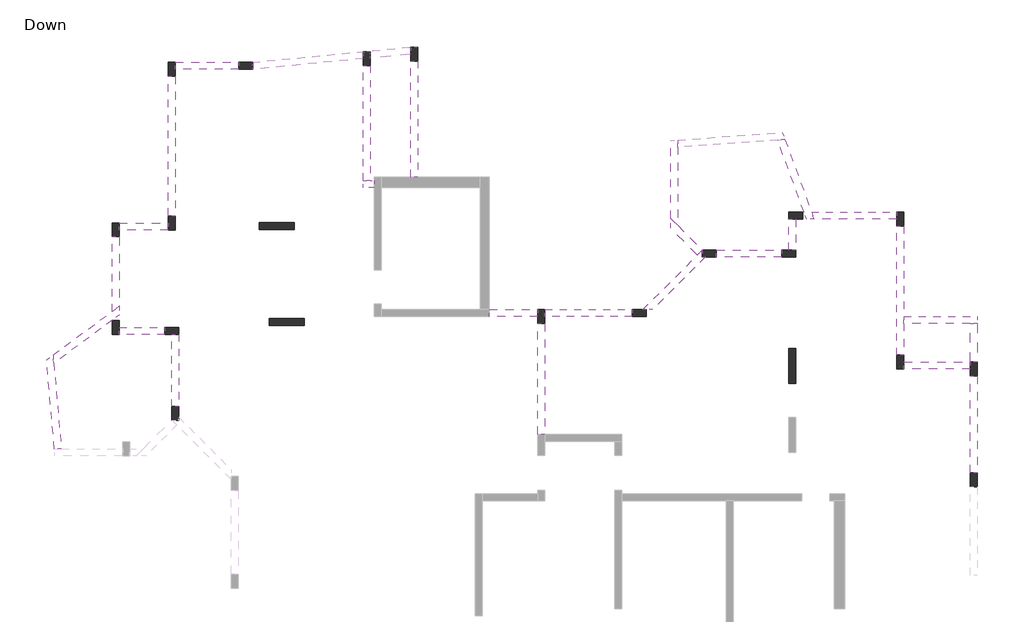
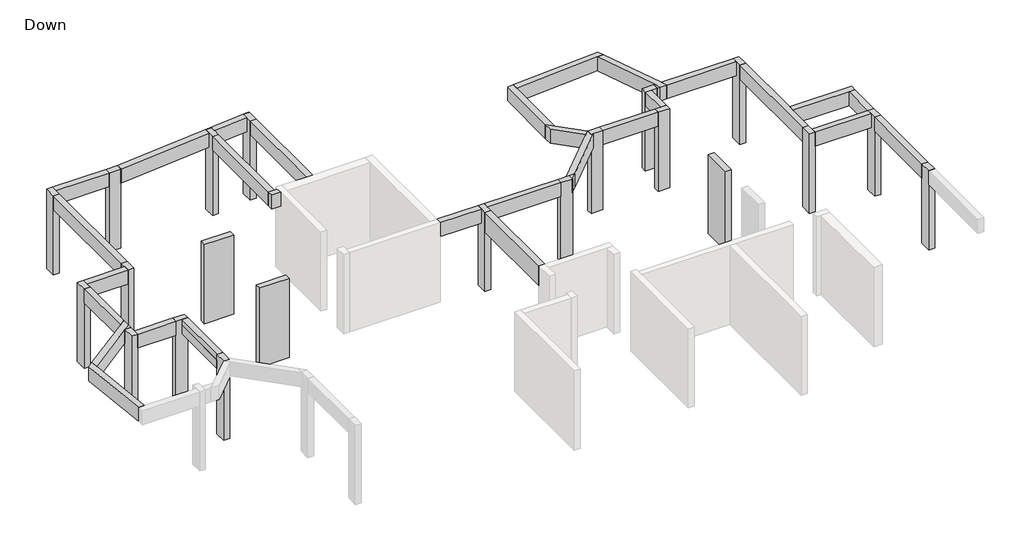
# One storey, part 3 of 3: 28 beams, 21 columns.
# Revit data of these elements (continued)
# Element 43 (IfcColumn, "Concrete Rectengular Column : 20/40") (continued)
#   Materials on its faces: "Concrete"
# Element 44 (IfcColumn, "Concrete Rectengular Column : 20/40")
#   Comments = ""
#   Mark = "C42"
#   SOFiSTiK_AMG_Comments = ""
#   SOFiSTiK_AMG_Scheduled = yes
#   SOFiSTiK_AMG_Adjusted = yes
#   Structural Material = Concrete
#   Phase Created = New Construction
#   Materials on its faces: "Concrete"
# Element 45 (IfcColumn, "Concrete Rectengular Column : 20/40")
#   Comments = ""
#   Mark = "C43"
#   SOFiSTiK_AMG_Comments = ""
#   SOFiSTiK_AMG_Scheduled = yes
#   SOFiSTiK_AMG_Adjusted = yes
#   Structural Material = Concrete
#   Phase Created = New Construction
#   Materials on its faces: "Concrete"
# Element 46 (IfcColumn, "Concrete Rectengular Column : 20/40")
#   Comments = ""
#   Mark = "C44"
#   SOFiSTiK_AMG_Comments = ""
#   SOFiSTiK_AMG_Scheduled = yes
#   SOFiSTiK_AMG_Adjusted = yes
#   Structural Material = Concrete
#   Phase Created = New Construction
#   Materials on its faces: "Concrete"
# Element 47 (IfcColumn, "Concrete Rectengular Column : 20/40")
#   Comments = ""
#   Mark = "C45"
#   SOFiSTiK_AMG_Comments = ""
#   SOFiSTiK_AMG_Scheduled = yes
#   SOFiSTiK_AMG_Adjusted = yes
#   Structural Material = Concrete
#   Phase Created = New Construction
#   Materials on its faces: "Concrete"
# Element 48 (IfcColumn, "Concrete Rectengular Column : 20/40")
#   Comments = ""
#   Mark = "C46"
#   SOFiSTiK_AMG_Comments = ""
#   SOFiSTiK_AMG_Scheduled = yes
#   SOFiSTiK_AMG_Adjusted = yes
#   Structural Material = Concrete
#   Phase Created = New Construction
#   Materials on its faces: "Concrete"
# Element 49 (IfcColumn, "Concrete Rectengular Column : 20/40")
#   Comments = ""
#   Mark = "C47"
#   SOFiSTiK_AMG_Comments = ""
#   SOFiSTiK_AMG_Scheduled = yes
#   SOFiSTiK_AMG_Adjusted = yes
#   Structural Material = Concrete
#   Phase Created = New Construction
#   Materials on its faces: "Concrete"
# Materials
#   "Concrete": class "Concrete", colour RGB 192 192 192, transparency 0, Keynote = "01000", Description = "Cast-in-place concrete", Cost = 0
